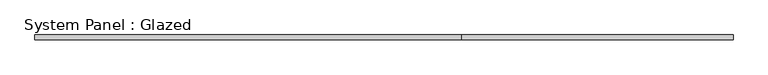
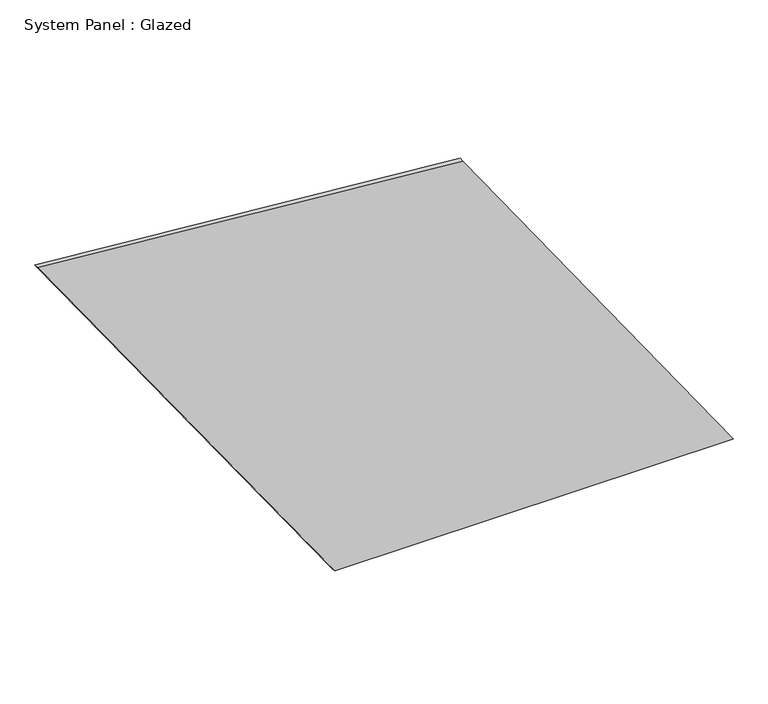
"""IFC4 building model written with IfcOpenShell, lengths in millimetres: plate geometry, System Panel : Glazed."""

import ifcopenshell
import ifcopenshell.guid

model = None  # the IFC model being written
_history = None  # IfcOwnerHistory: only IFC2X3 demands one
_inside = {}  # id of a spatial element -> (the spatial element, [elements in it])
_under = {}  # id of a project, library or spatial element -> (it, [spatial elements below it])
_declared = {}  # id of a project -> (the project, [libraries it declares])
_typed = {}  # id of a type object -> (the type object, [elements of that type])
_made_of = {}  # id of a material, layer set ... -> (it, [elements and type objects made of it])


def new_model(schema):
    """Start an empty IFC model of exactly this schema.

    Asked for "IFC4X3", IfcOpenShell would pick the latest addendum, in which some entities
    have other attributes; the version numbers below select the first issue.
    IFC2X3 requires an IfcOwnerHistory on every rooted entity: one is made here for all.
    """
    global model, _history
    if schema == "IFC4X3":
        model = ifcopenshell.file(schema_version=(4, 3, 0, 0))
    else:
        model = ifcopenshell.file(schema=schema)
    _inside.clear()
    _under.clear()
    _declared.clear()
    _typed.clear()
    _made_of.clear()
    _history = None
    if model.schema == "IFC2X3":
        org = make("IfcOrganization", Name="unknown")
        user = make(
            "IfcPersonAndOrganization",
            ThePerson=make("IfcPerson", FamilyName="unknown"),
            TheOrganization=org,
        )
        app = make(
            "IfcApplication",
            ApplicationDeveloper=org,
            Version="unknown",
            ApplicationFullName="unknown",
            ApplicationIdentifier="unknown",
        )
        _history = make(
            "IfcOwnerHistory",
            OwningUser=user,
            OwningApplication=app,
            ChangeAction="ADDED",
            CreationDate=0,
        )
    return model


def make(cls, **values):
    """One entity of the class cls with the attributes given. An attribute that is None is left unset."""
    return model.create_entity(
        cls, **{name: value for name, value in values.items() if value is not None}
    )


def rooted(cls, **values):
    """An entity with a GlobalId (a new one), such as an element, a storey or a relation."""
    return make(cls, GlobalId=ifcopenshell.guid.new(), OwnerHistory=_history, **values)


def si_unit(unit_type, name, prefix=None):
    """IfcSIUnit, for example si_unit("LENGTHUNIT", "METRE", prefix="MILLI")."""
    return make("IfcSIUnit", UnitType=unit_type, Prefix=prefix, Name=name)


def assignment(units):
    """IfcUnitAssignment: the units of a project."""
    return None if units is None else make("IfcUnitAssignment", Units=units)


def point(xyz):
    """IfcCartesianPoint."""
    return None if xyz is None else make("IfcCartesianPoint", Coordinates=xyz)


def direction(xyz):
    """IfcDirection."""
    return None if xyz is None else make("IfcDirection", DirectionRatios=xyz)


def frame(location, z_axis=None, x_axis=None):
    """IfcAxis2Placement3D, a coordinate frame: its origin and axes. An axis left out is left unset."""
    return make(
        "IfcAxis2Placement3D",
        Location=point(location),
        Axis=direction(z_axis),
        RefDirection=direction(x_axis),
    )


def origin():
    """The frame at (0, 0, 0) with its axes left unset."""
    return frame((0.0, 0.0, 0.0))


def place(relative_to, where):
    """IfcLocalPlacement: puts the frame where relative to a parent placement (None: the world)."""
    return make(
        "IfcLocalPlacement", PlacementRelTo=relative_to, RelativePlacement=where
    )


def context(
    kind, dimensions, precision=None, world=None, true_north=None, identifier=None
):
    """IfcGeometricRepresentationContext, for example the 3D "Model" context."""
    return make(
        "IfcGeometricRepresentationContext",
        ContextIdentifier=identifier,
        ContextType=kind,
        CoordinateSpaceDimension=dimensions,
        Precision=precision,
        WorldCoordinateSystem=world,
        TrueNorth=true_north,
    )


def project(units=None, contexts=None):
    """IfcProject with its units and contexts."""
    return rooted(
        "IfcProject",
        Name="project",
        RepresentationContexts=contexts,
        UnitsInContext=assignment(units),
    )


def spatial(cls, under=None, at=None, **own):
    """A site, building, storey or space (cls), placed at a placement, below another one or the project."""
    s = rooted(cls, ObjectPlacement=at, **own)
    if under is not None:
        _under.setdefault(under.id(), (under, []))[1].append(s)
    return s


def polyline(points):
    """IfcPolyline through the points."""
    return make("IfcPolyline", Points=[point(p) for p in points])


def outline(outer, holes=None, kind="AREA"):
    """IfcArbitraryClosedProfileDef: a profile drawn as a closed curve; with holes, ...WithVoids."""
    if holes is None:
        return make("IfcArbitraryClosedProfileDef", ProfileType=kind, OuterCurve=outer)
    return make(
        "IfcArbitraryProfileDefWithVoids",
        ProfileType=kind,
        OuterCurve=outer,
        InnerCurves=holes,
    )


def extrude(swept, where, along, depth):
    """IfcExtrudedAreaSolid: the profile swept, set in the frame where, extruded along a direction by depth."""
    return make(
        "IfcExtrudedAreaSolid",
        SweptArea=swept,
        Position=where,
        ExtrudedDirection=direction(along),
        Depth=depth,
    )


def shape(context_of_items, identifier, shape_type, items):
    """IfcShapeRepresentation: the items that make up one representation, for example the "Body"."""
    return make(
        "IfcShapeRepresentation",
        ContextOfItems=context_of_items,
        RepresentationIdentifier=identifier,
        RepresentationType=shape_type,
        Items=items,
    )


def source(mapping_origin, context_of_items, identifier, shape_type, items):
    """IfcRepresentationMap: a shape defined once, which mapped items show again and again."""
    return make(
        "IfcRepresentationMap",
        MappingOrigin=mapping_origin,
        MappedRepresentation=shape(context_of_items, identifier, shape_type, items),
    )


def transform(
    local_origin,
    x_axis=None,
    y_axis=None,
    z_axis=None,
    scale=None,
    scale2=None,
    scale3=None,
    uniform=True,
):
    """IfcCartesianTransformationOperator3D, or its non-uniform kind. x_axis, y_axis, z_axis: its Axis1, 2, 3."""
    if uniform:
        return make(
            "IfcCartesianTransformationOperator3D",
            Axis1=direction(x_axis),
            Axis2=direction(y_axis),
            LocalOrigin=point(local_origin),
            Scale=scale,
            Axis3=direction(z_axis),
        )
    return make(
        "IfcCartesianTransformationOperator3DnonUniform",
        Axis1=direction(x_axis),
        Axis2=direction(y_axis),
        LocalOrigin=point(local_origin),
        Scale=scale,
        Axis3=direction(z_axis),
        Scale2=scale2,
        Scale3=scale3,
    )


def mapped(mapping_source, mapping_target):
    """IfcMappedItem: shows the shape of a source again, moved by a transform."""
    return make(
        "IfcMappedItem", MappingSource=mapping_source, MappingTarget=mapping_target
    )


def made_of(thing, what):
    """Note that an element or type object is made of a material, layer set ...; save() writes the relation."""
    if what is not None:
        _made_of.setdefault(what.id(), (what, []))[1].append(thing)
    return thing


def element(
    cls,
    number,
    at=None,
    inside=None,
    cuts=None,
    type_object=None,
    material=None,
    context=None,
    identifier="Body",
    shape_type=None,
    held_by="IfcProductDefinitionShape",
    body=None,
    shapes=None,
    **own,
):
    """One element of the class cls, such as IfcWall. Its Tag is "e" and its number.

    at: its placement. inside: the storey or other place that contains it. cuts: it is an
    opening in that element (IfcRelVoidsElement). A single representation is given by context,
    identifier, shape_type and body (its items); several are given by shapes. held_by: the class
    of the entity that holds the representations. save() writes the other relations.
    """
    e = rooted(cls, Tag="e%d" % number, ObjectPlacement=at, **own)
    if body is not None:
        shapes = [shape(context, identifier, shape_type, body)]
    if shapes is not None:
        e.Representation = make(held_by, Representations=shapes)
    if inside is not None:
        _inside.setdefault(inside.id(), (inside, []))[1].append(e)
    if cuts is not None:
        rooted(
            "IfcRelVoidsElement", RelatingBuildingElement=cuts, RelatedOpeningElement=e
        )
    if type_object is not None:
        _typed.setdefault(type_object.id(), (type_object, []))[1].append(e)
    return made_of(e, material)


def aggregate(whole, parts):
    """IfcRelAggregates: a whole, such as a stair, and the parts it consists of."""
    return rooted("IfcRelAggregates", RelatingObject=whole, RelatedObjects=parts)


def save(model, path):
    """Write the relations noted so far, then the file.

    IfcRelAggregates (storeys below a building ...), IfcRelContainedInSpatialStructure (elements
    in a storey), IfcRelDefinesByType, IfcRelAssociatesMaterial and IfcRelDeclares: one each for
    every whole, place, type object, material and project.
    """
    for whole, parts in _under.values():
        aggregate(whole, parts)
    for where, things in _inside.values():
        rooted(
            "IfcRelContainedInSpatialStructure",
            RelatedElements=things,
            RelatingStructure=where,
        )
    for kind, things in _typed.values():
        rooted("IfcRelDefinesByType", RelatedObjects=things, RelatingType=kind)
    for what, things in _made_of.values():
        rooted("IfcRelAssociatesMaterial", RelatedObjects=things, RelatingMaterial=what)
    for by, libraries in _declared.values():
        rooted("IfcRelDeclares", RelatingContext=by, RelatedDefinitions=libraries)
    model.write(path)


def system_panel_glazed_e0448721(model_context):
    return source(origin(), model_context, "Body", "SweptSolid", [
        extrude(outline(polyline([(0.0, -268.47988), (0.0, 1840.2925101), (2057.7653992, 409.9882177), (2247.4031732, -1840.2925101), (0.0, -268.47988)])), frame((0.0, -49.5, 0.0), z_axis=(0.0, 1.0, 0.0), x_axis=(0.0, 0.0, 1.0)), (0.0, 0.0, 1.0), 25.0),
    ])


if __name__ == "__main__":
    model = new_model("IFC4")
    model_context = context("Model", 3, world=origin())
    ifc_project = project(units=[si_unit("LENGTHUNIT", "METRE", prefix="MILLI")], contexts=[model_context])
    site = spatial("IfcSite", under=ifc_project)
    building = spatial("IfcBuilding", under=site)
    placement = place(None, origin())
    system_panel_glazed_shape = system_panel_glazed_e0448721(model_context)
    element("IfcPlate", 1, ObjectType="System Panel : Glazed", at=placement, inside=building, context=model_context, shape_type="MappedRepresentation", body=[
        mapped(system_panel_glazed_shape, transform((0.0, 0.0, 0.0), x_axis=(1.0, 0.0, 0.0), y_axis=(0.0, 1.0, 0.0), z_axis=(0.0, 0.0, 1.0))),
    ])
    save(model, "model.ifc")

# Revit data of these elements
# Element 1 (IfcPlate, "System Panel : Glazed")
#   Materials on its faces: "Glass, Clear Glazing"
# Materials
#   "Glass, Clear Glazing": class "Glass", colour RGB 247 249 248, transparency 0.85, Description = "Clear glazing", Cost = 0
